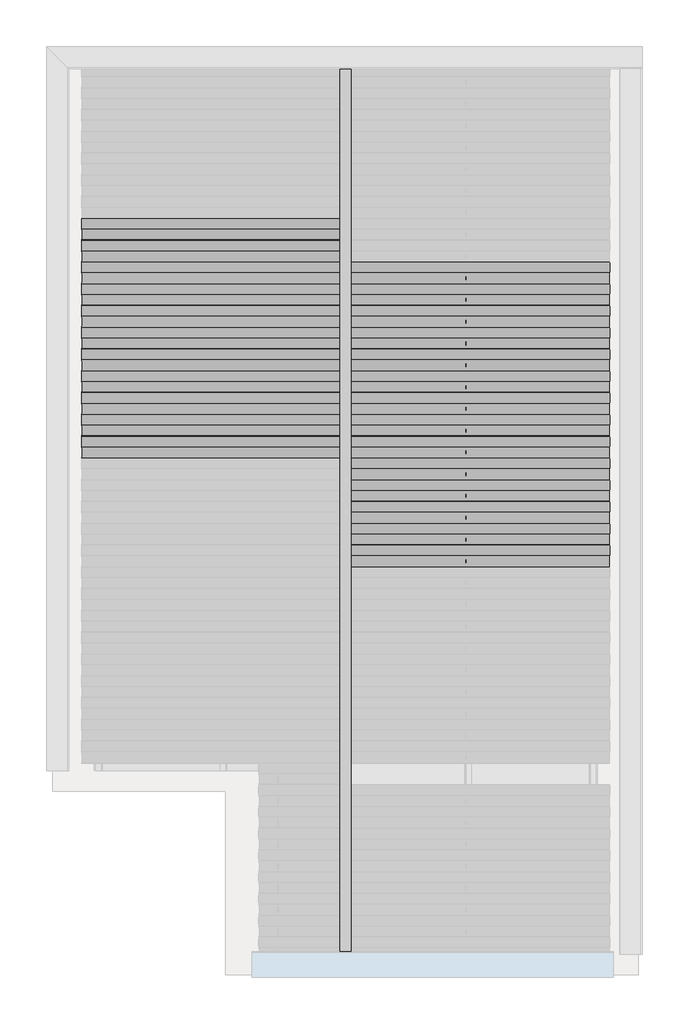
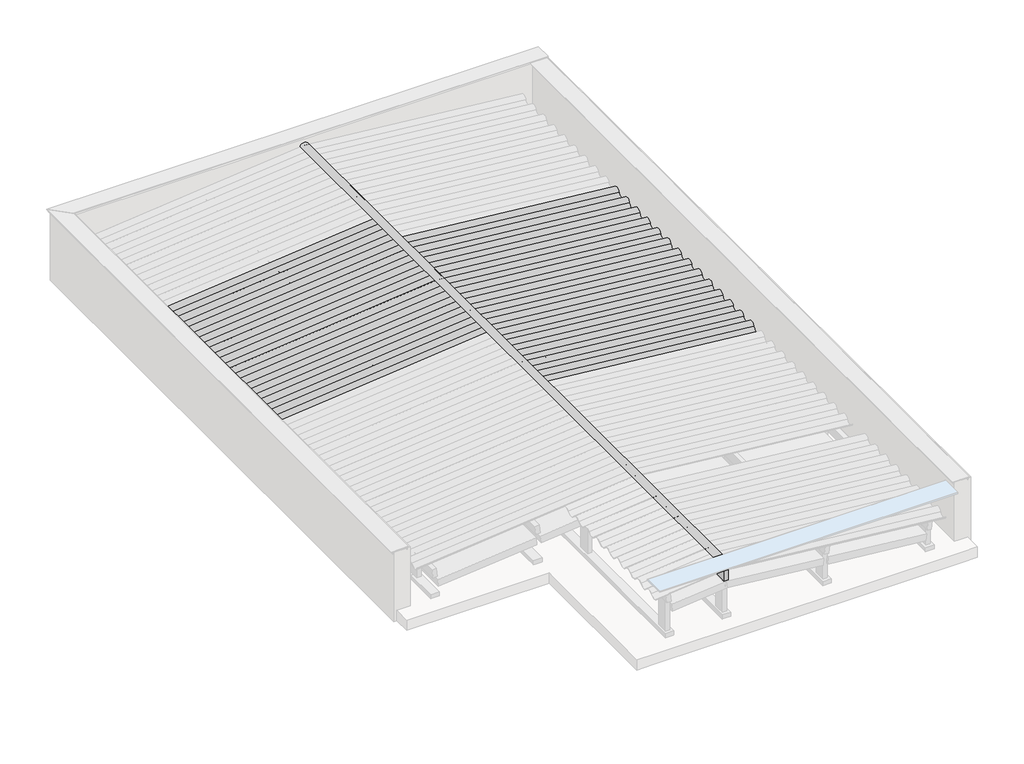
# One storey, part 3 of 4: 34 beams, 8 columns.
"""IFC4 building model written with IfcOpenShell, lengths in millimetres."""

import ifcopenshell
import ifcopenshell.guid

model = None  # the IFC model being written
_history = None  # IfcOwnerHistory: only IFC2X3 demands one
_inside = {}  # id of a spatial element -> (the spatial element, [elements in it])
_under = {}  # id of a project, library or spatial element -> (it, [spatial elements below it])
_declared = {}  # id of a project -> (the project, [libraries it declares])
_typed = {}  # id of a type object -> (the type object, [elements of that type])
_made_of = {}  # id of a material, layer set ... -> (it, [elements and type objects made of it])


def new_model(schema):
    """Start an empty IFC model of exactly this schema.

    Asked for "IFC4X3", IfcOpenShell would pick the latest addendum, in which some entities
    have other attributes; the version numbers below select the first issue.
    IFC2X3 requires an IfcOwnerHistory on every rooted entity: one is made here for all.
    """
    global model, _history
    if schema == "IFC4X3":
        model = ifcopenshell.file(schema_version=(4, 3, 0, 0))
    else:
        model = ifcopenshell.file(schema=schema)
    _inside.clear()
    _under.clear()
    _declared.clear()
    _typed.clear()
    _made_of.clear()
    _history = None
    if model.schema == "IFC2X3":
        org = make("IfcOrganization", Name="unknown")
        user = make(
            "IfcPersonAndOrganization",
            ThePerson=make("IfcPerson", FamilyName="unknown"),
            TheOrganization=org,
        )
        app = make(
            "IfcApplication",
            ApplicationDeveloper=org,
            Version="unknown",
            ApplicationFullName="unknown",
            ApplicationIdentifier="unknown",
        )
        _history = make(
            "IfcOwnerHistory",
            OwningUser=user,
            OwningApplication=app,
            ChangeAction="ADDED",
            CreationDate=0,
        )
    return model


def make(cls, **values):
    """One entity of the class cls with the attributes given. An attribute that is None is left unset."""
    return model.create_entity(
        cls, **{name: value for name, value in values.items() if value is not None}
    )


def rooted(cls, **values):
    """An entity with a GlobalId (a new one), such as an element, a storey or a relation."""
    return make(cls, GlobalId=ifcopenshell.guid.new(), OwnerHistory=_history, **values)


def si_unit(unit_type, name, prefix=None):
    """IfcSIUnit, for example si_unit("LENGTHUNIT", "METRE", prefix="MILLI")."""
    return make("IfcSIUnit", UnitType=unit_type, Prefix=prefix, Name=name)


def assignment(units):
    """IfcUnitAssignment: the units of a project."""
    return None if units is None else make("IfcUnitAssignment", Units=units)


def point(xyz):
    """IfcCartesianPoint."""
    return None if xyz is None else make("IfcCartesianPoint", Coordinates=xyz)


def direction(xyz):
    """IfcDirection."""
    return None if xyz is None else make("IfcDirection", DirectionRatios=xyz)


def frame(location, z_axis=None, x_axis=None):
    """IfcAxis2Placement3D, a coordinate frame: its origin and axes. An axis left out is left unset."""
    return make(
        "IfcAxis2Placement3D",
        Location=point(location),
        Axis=direction(z_axis),
        RefDirection=direction(x_axis),
    )


def frame_2d(location, x_axis=None):
    """IfcAxis2Placement2D, a coordinate frame in the plane: its origin and x axis."""
    return make(
        "IfcAxis2Placement2D", Location=point(location), RefDirection=direction(x_axis)
    )


def origin():
    """The frame at (0, 0, 0) with its axes left unset."""
    return frame((0.0, 0.0, 0.0))


def place(relative_to, where):
    """IfcLocalPlacement: puts the frame where relative to a parent placement (None: the world)."""
    return make(
        "IfcLocalPlacement", PlacementRelTo=relative_to, RelativePlacement=where
    )


def context(
    kind, dimensions, precision=None, world=None, true_north=None, identifier=None
):
    """IfcGeometricRepresentationContext, for example the 3D "Model" context."""
    return make(
        "IfcGeometricRepresentationContext",
        ContextIdentifier=identifier,
        ContextType=kind,
        CoordinateSpaceDimension=dimensions,
        Precision=precision,
        WorldCoordinateSystem=world,
        TrueNorth=true_north,
    )


def project(units=None, contexts=None):
    """IfcProject with its units and contexts."""
    return rooted(
        "IfcProject",
        Name="project",
        RepresentationContexts=contexts,
        UnitsInContext=assignment(units),
    )


def spatial(cls, under=None, at=None, **own):
    """A site, building, storey or space (cls), placed at a placement, below another one or the project."""
    s = rooted(cls, ObjectPlacement=at, **own)
    if under is not None:
        _under.setdefault(under.id(), (under, []))[1].append(s)
    return s


def polyline(points):
    """IfcPolyline through the points."""
    return make("IfcPolyline", Points=[point(p) for p in points])


def circle_curve(where, radius):
    """IfcCircle in the frame where."""
    return make("IfcCircle", Position=where, Radius=radius)


def trimmed(basis, trim1, trim2, sense, master):
    """IfcTrimmedCurve: the piece of a basis curve between two trims."""
    return make(
        "IfcTrimmedCurve",
        BasisCurve=basis,
        Trim1=trim1,
        Trim2=trim2,
        SenseAgreement=sense,
        MasterRepresentation=master,
    )


def segment(curve, same_sense, transition):
    """IfcCompositeCurveSegment."""
    return make(
        "IfcCompositeCurveSegment",
        Transition=transition,
        SameSense=same_sense,
        ParentCurve=curve,
    )


def composite_curve(segments, self_intersect=None):
    """IfcCompositeCurve: segments joined end to end."""
    return make("IfcCompositeCurve", Segments=segments, SelfIntersect=self_intersect)


def outline(outer, holes=None, kind="AREA"):
    """IfcArbitraryClosedProfileDef: a profile drawn as a closed curve; with holes, ...WithVoids."""
    if holes is None:
        return make("IfcArbitraryClosedProfileDef", ProfileType=kind, OuterCurve=outer)
    return make(
        "IfcArbitraryProfileDefWithVoids",
        ProfileType=kind,
        OuterCurve=outer,
        InnerCurves=holes,
    )


def extrude(swept, where, along, depth):
    """IfcExtrudedAreaSolid: the profile swept, set in the frame where, extruded along a direction by depth."""
    return make(
        "IfcExtrudedAreaSolid",
        SweptArea=swept,
        Position=where,
        ExtrudedDirection=direction(along),
        Depth=depth,
    )


def shape(context_of_items, identifier, shape_type, items):
    """IfcShapeRepresentation: the items that make up one representation, for example the "Body"."""
    return make(
        "IfcShapeRepresentation",
        ContextOfItems=context_of_items,
        RepresentationIdentifier=identifier,
        RepresentationType=shape_type,
        Items=items,
    )


def source(mapping_origin, context_of_items, identifier, shape_type, items):
    """IfcRepresentationMap: a shape defined once, which mapped items show again and again."""
    return make(
        "IfcRepresentationMap",
        MappingOrigin=mapping_origin,
        MappedRepresentation=shape(context_of_items, identifier, shape_type, items),
    )


def transform(
    local_origin,
    x_axis=None,
    y_axis=None,
    z_axis=None,
    scale=None,
    scale2=None,
    scale3=None,
    uniform=True,
):
    """IfcCartesianTransformationOperator3D, or its non-uniform kind. x_axis, y_axis, z_axis: its Axis1, 2, 3."""
    if uniform:
        return make(
            "IfcCartesianTransformationOperator3D",
            Axis1=direction(x_axis),
            Axis2=direction(y_axis),
            LocalOrigin=point(local_origin),
            Scale=scale,
            Axis3=direction(z_axis),
        )
    return make(
        "IfcCartesianTransformationOperator3DnonUniform",
        Axis1=direction(x_axis),
        Axis2=direction(y_axis),
        LocalOrigin=point(local_origin),
        Scale=scale,
        Axis3=direction(z_axis),
        Scale2=scale2,
        Scale3=scale3,
    )


def mapped(mapping_source, mapping_target):
    """IfcMappedItem: shows the shape of a source again, moved by a transform."""
    return make(
        "IfcMappedItem", MappingSource=mapping_source, MappingTarget=mapping_target
    )


def made_of(thing, what):
    """Note that an element or type object is made of a material, layer set ...; save() writes the relation."""
    if what is not None:
        _made_of.setdefault(what.id(), (what, []))[1].append(thing)
    return thing


def element(
    cls,
    number,
    at=None,
    inside=None,
    cuts=None,
    type_object=None,
    material=None,
    context=None,
    identifier="Body",
    shape_type=None,
    held_by="IfcProductDefinitionShape",
    body=None,
    shapes=None,
    **own,
):
    """One element of the class cls, such as IfcWall. Its Tag is "e" and its number.

    at: its placement. inside: the storey or other place that contains it. cuts: it is an
    opening in that element (IfcRelVoidsElement). A single representation is given by context,
    identifier, shape_type and body (its items); several are given by shapes. held_by: the class
    of the entity that holds the representations. save() writes the other relations.
    """
    e = rooted(cls, Tag="e%d" % number, ObjectPlacement=at, **own)
    if body is not None:
        shapes = [shape(context, identifier, shape_type, body)]
    if shapes is not None:
        e.Representation = make(held_by, Representations=shapes)
    if inside is not None:
        _inside.setdefault(inside.id(), (inside, []))[1].append(e)
    if cuts is not None:
        rooted(
            "IfcRelVoidsElement", RelatingBuildingElement=cuts, RelatedOpeningElement=e
        )
    if type_object is not None:
        _typed.setdefault(type_object.id(), (type_object, []))[1].append(e)
    return made_of(e, material)


def aggregate(whole, parts):
    """IfcRelAggregates: a whole, such as a stair, and the parts it consists of."""
    return rooted("IfcRelAggregates", RelatingObject=whole, RelatedObjects=parts)


def save(model, path):
    """Write the relations noted so far, then the file.

    IfcRelAggregates (storeys below a building ...), IfcRelContainedInSpatialStructure (elements
    in a storey), IfcRelDefinesByType, IfcRelAssociatesMaterial and IfcRelDeclares: one each for
    every whole, place, type object, material and project.
    """
    for whole, parts in _under.values():
        aggregate(whole, parts)
    for where, things in _inside.values():
        rooted(
            "IfcRelContainedInSpatialStructure",
            RelatedElements=things,
            RelatingStructure=where,
        )
    for kind, things in _typed.values():
        rooted("IfcRelDefinesByType", RelatedObjects=things, RelatingType=kind)
    for what, things in _made_of.values():
        rooted("IfcRelAssociatesMaterial", RelatedObjects=things, RelatingMaterial=what)
    for by, libraries in _declared.values():
        rooted("IfcRelDeclares", RelatingContext=by, RelatedDefinitions=libraries)
    model.write(path)


def cumeeira_telha_ondulada_fibrocimento_c9eafb3e(model_context):
    return source(origin(), model_context, "Body", "SweptSolid", [
        extrude(outline(composite_curve([segment(polyline([(58.3970135, 42.4437972), (53.9055884, 40.2467307)]), True, "CONTINUOUS"), segment(trimmed(circle_curve(frame_2d((-1.6029865, 13.0936483)), 61.7939461), [point((53.9055884, 40.2467307))], [point((-57.1115615, 40.2467307))], True, "CARTESIAN"), True, "CONTINUOUS"), segment(polyline([(-57.1115615, 40.2467307), (-61.6029865, 42.4437972)]), True, "CONTINUOUS"), segment(trimmed(circle_curve(frame_2d((-1.6029865, 13.0936483)), 66.7939461), [point((-61.6029865, 42.4437972))], [point((58.3970135, 42.4437972))], False, "CARTESIAN"), True, "CONTINUOUS")], self_intersect=False)), frame((-4969.5, 0.0, 0.0), z_axis=(1.0, 0.0, 0.0), x_axis=(0.0, 1.0, 0.0)), (0.0, 0.0, 1.0), 9939.0),
    ])


def viga_cumeeira_6x16cm_10b61863(model_context):
    return source(origin(), model_context, "Body", "SweptSolid", [
        extrude(outline(polyline([(4969.4999994, 30.0), (4969.4999994, -30.0), (-4969.4999994, -30.0), (-4969.4999994, 30.0), (4969.4999994, 30.0)])), frame((0.0, 0.0, -80.0), z_axis=(0.0, 0.0, 1.0), x_axis=(1.0, 0.0, 0.0)), (0.0, 0.0, 1.0), 160.0),
    ])


def column_7d6827b5(model_context):
    return source(origin(), model_context, "Body", "SweptSolid", [
        extrude(outline(polyline([(30.0, 80.0), (30.0, -80.0), (-30.0, -80.0), (-30.0, 80.0), (30.0, 80.0)])), frame((0.0, 0.0, 4460.0), z_axis=(0.0, 0.0, 1.0), x_axis=(1.0, 0.0, 0.0)), (0.0, 0.0, 1.0), 466.0),
    ])


def column_c7348c99(model_context):
    return source(origin(), model_context, "Body", "SweptSolid", [
        extrude(outline(polyline([(30.0, 80.0), (30.0, -80.0), (-30.0, -80.0), (-30.0, 80.0), (30.0, 80.0)])), frame((0.0, 0.0, 4460.0), z_axis=(0.0, 0.0, 1.0), x_axis=(1.0, 0.0, 0.0)), (0.0, 0.0, 1.0), 372.8),
    ])


def column_6cc9e01b(model_context):
    return source(origin(), model_context, "Body", "SweptSolid", [
        extrude(outline(polyline([(30.0, 80.0), (30.0, -80.0), (-30.0, -80.0), (-30.0, 80.0), (30.0, 80.0)])), frame((0.0, 0.0, 4460.0), z_axis=(0.0, 0.0, 1.0), x_axis=(1.0, 0.0, 0.0)), (0.0, 0.0, 1.0), 233.0),
    ])


model = new_model("IFC4")

# Units and contexts
model_context = context("Model", 3, world=origin())
ifc_project = project(units=[si_unit("LENGTHUNIT", "METRE", prefix="MILLI")], contexts=[model_context])

# Site, building, storey
site = spatial("IfcSite", under=ifc_project)
building = spatial("IfcBuilding", under=site)
storey = spatial("IfcBuildingStorey", under=building, Name="COB. SALA ESTAR", Elevation=4400.0)

# Beams
placement = place(None, origin())
element("IfcBeam", 1, ObjectType="Madeira de lei : Berço 6x12cm", at=placement, inside=storey, context=model_context, shape_type="SweptSolid", body=[
    extrude(outline(polyline([(-3400.8557491, 2180.4300147), (-3280.8557491, 2180.4300147), (-3280.8557491, 180.4300153), (-3400.8557491, 180.4300153), (-3400.8557491, 2180.4300147)])), frame((0.0, 0.0, 4400.0), z_axis=(0.0, 0.0, 1.0), x_axis=(1.0, 0.0, 0.0)), (0.0, 0.0, 1.0), 60.0),
])
element("IfcBeam", 2, ObjectType="Madeira de lei : Berço 6x12cm", at=placement, inside=storey, context=model_context, shape_type="SweptSolid", body=[
    extrude(outline(polyline([(-3400.8557491, 4180.4300153), (-3280.8557491, 4180.4300153), (-3280.8557491, 2180.4300159), (-3400.8557491, 2180.4300159), (-3400.8557491, 4180.4300153)])), frame((0.0, 0.0, 4400.0), z_axis=(0.0, 0.0, 1.0), x_axis=(1.0, 0.0, 0.0)), (0.0, 0.0, 1.0), 60.0),
])
element("IfcBeam", 3, ObjectType="Madeira de lei : Berço 6x12cm", at=placement, inside=storey, context=model_context, shape_type="SweptSolid", body=[
    extrude(outline(polyline([(-2032.3324227, 2180.4300147), (-1912.3324227, 2180.4300147), (-1912.3324227, 180.4300153), (-2032.3324227, 180.4300153), (-2032.3324227, 2180.4300147)])), frame((0.0, 0.0, 4400.0), z_axis=(0.0, 0.0, 1.0), x_axis=(1.0, 0.0, 0.0)), (0.0, 0.0, 1.0), 60.0),
])
element("IfcBeam", 4, ObjectType="Madeira de lei : Berço 6x12cm", at=placement, inside=storey, context=model_context, shape_type="SweptSolid", body=[
    extrude(outline(polyline([(-634.0324227, 2180.4300147), (-514.0324227, 2180.4300147), (-514.0324227, 180.4300153), (-634.0324227, 180.4300153), (-634.0324227, 2180.4300147)])), frame((0.0, 0.0, 4400.0), z_axis=(0.0, 0.0, 1.0), x_axis=(1.0, 0.0, 0.0)), (0.0, 0.0, 1.0), 60.0),
])
element("IfcBeam", 5, ObjectType="Madeira de lei : Berço 6x12cm", at=placement, inside=storey, context=model_context, shape_type="SweptSolid", body=[
    extrude(outline(polyline([(-6167.5301913, 4180.4300153), (-6047.5301913, 4180.4300153), (-6047.5301913, 2180.4300159), (-6167.5301913, 2180.4300159), (-6167.5301913, 4180.4300153)])), frame((0.0, 0.0, 4400.0), z_axis=(0.0, 0.0, 1.0), x_axis=(1.0, 0.0, 0.0)), (0.0, 0.0, 1.0), 60.0),
])
element("IfcBeam", 6, ObjectType="Madeira de lei : Berço 6x12cm", at=placement, inside=storey, context=model_context, shape_type="SweptSolid", body=[
    extrude(outline(polyline([(-4769.2301913, 2180.4300147), (-4649.2301913, 2180.4300147), (-4649.2301913, 180.4300153), (-4769.2301913, 180.4300153), (-4769.2301913, 2180.4300147)])), frame((0.0, 0.0, 4400.0), z_axis=(0.0, 0.0, 1.0), x_axis=(1.0, 0.0, 0.0)), (0.0, 0.0, 1.0), 60.0),
])
element("IfcBeam", 7, ObjectType="Madeira de lei : Berço 6x12cm", at=placement, inside=storey, context=model_context, shape_type="SweptSolid", body=[
    extrude(outline(polyline([(-4769.2301913, 4180.4300153), (-4649.2301913, 4180.4300153), (-4649.2301913, 2180.4300159), (-4769.2301913, 2180.4300159), (-4769.2301913, 4180.4300153)])), frame((0.0, 0.0, 4400.0), z_axis=(0.0, 0.0, 1.0), x_axis=(1.0, 0.0, 0.0)), (0.0, 0.0, 1.0), 60.0),
])
cumeeira_telha_ondulada_fibrocimento_shape = cumeeira_telha_ondulada_fibrocimento_c9eafb3e(model_context)
element("IfcBeam", 8, ObjectType="Cumeeira Telha Ondulada : Fibrocimento", at=placement, inside=storey, context=model_context, shape_type="MappedRepresentation", body=[
    mapped(cumeeira_telha_ondulada_fibrocimento_shape, transform((-3340.8557491, 623.9300153, 5123.1251229), x_axis=(0.0, -1.0, 0.0), y_axis=(1.0, 0.0, 0.0), z_axis=(0.0, 0.0, 1.0))),
])
element("IfcBeam", 9, ObjectType="Telha Ondulada : Fibrocimento", at=placement, inside=storey, context=model_context, shape_type="SweptSolid", body=[
    extrude(outline(composite_curve([segment(trimmed(circle_curve(frame_2d((-58.7002978, -53.2060538)), 66.7939461), [point((-29.3501489, 6.7939462))], [point((-29.3501489, -113.2060538))], False, "CARTESIAN"), True, "CONTINUOUS"), segment(polyline([(-29.3501489, -113.2060538), (-31.5472154, -108.7146288)]), True, "CONTINUOUS"), segment(trimmed(circle_curve(frame_2d((-58.7002978, -53.2060538)), 61.7939461), [point((-31.5472154, -108.7146288))], [point((-31.5472154, 2.3025211))], True, "CARTESIAN"), True, "CONTINUOUS"), segment(trimmed(circle_curve(frame_2d((0.0, 66.7939462)), 71.7939461), [point((-31.5472154, 2.3025211))], [point((-31.5472154, 131.2853712))], False, "CARTESIAN"), True, "CONTINUOUS"), segment(polyline([(-31.5472154, 131.2853712), (-29.3501489, 126.7939462)]), True, "CONTINUOUS"), segment(trimmed(circle_curve(frame_2d((0.0, 66.7939462)), 66.7939461), [point((-29.3501489, 126.7939462))], [point((-29.3501489, 6.7939462))], True, "CARTESIAN"), True, "CONTINUOUS")], self_intersect=False)), frame((-6307.6707245, 1355.826948, 4862.7215886), z_axis=(0.9950371902099892, 0.0, 0.09950371902099969), x_axis=(-0.09950371902099969, 0.0, 0.9950371902099892)), (0.0, 0.0, 1.0), 2972.5075682),
])
element("IfcBeam", 10, ObjectType="Telha Ondulada : Fibrocimento", at=placement, inside=storey, context=model_context, shape_type="SweptSolid", body=[
    extrude(outline(composite_curve([segment(trimmed(circle_curve(frame_2d((-58.7002978, -53.2060538)), 66.7939461), [point((-29.3501489, 6.7939462))], [point((-29.3501489, -113.2060538))], False, "CARTESIAN"), True, "CONTINUOUS"), segment(polyline([(-29.3501489, -113.2060538), (-31.5472154, -108.7146288)]), True, "CONTINUOUS"), segment(trimmed(circle_curve(frame_2d((-58.7002978, -53.2060538)), 61.7939461), [point((-31.5472154, -108.7146288))], [point((-31.5472154, 2.3025211))], True, "CARTESIAN"), True, "CONTINUOUS"), segment(trimmed(circle_curve(frame_2d((0.0, 66.7939462)), 71.7939461), [point((-31.5472154, 2.3025211))], [point((-31.5472154, 131.2853712))], False, "CARTESIAN"), True, "CONTINUOUS"), segment(polyline([(-31.5472154, 131.2853712), (-29.3501489, 126.7939462)]), True, "CONTINUOUS"), segment(trimmed(circle_curve(frame_2d((0.0, 66.7939462)), 66.7939461), [point((-29.3501489, 126.7939462))], [point((-29.3501489, 6.7939462))], True, "CARTESIAN"), True, "CONTINUOUS")], self_intersect=False)), frame((-6307.6707245, 1600.326948, 4862.7215886), z_axis=(0.9950371902099892, 0.0, 0.09950371902099972), x_axis=(-0.09950371902099972, 0.0, 0.9950371902099892)), (0.0, 0.0, 1.0), 2972.5075682),
])
element("IfcBeam", 11, ObjectType="Telha Ondulada : Fibrocimento", at=placement, inside=storey, context=model_context, shape_type="SweptSolid", body=[
    extrude(outline(composite_curve([segment(trimmed(circle_curve(frame_2d((-58.7002978, -53.2060538)), 66.7939461), [point((-29.3501489, 6.7939462))], [point((-29.3501489, -113.2060538))], False, "CARTESIAN"), True, "CONTINUOUS"), segment(polyline([(-29.3501489, -113.2060538), (-31.5472154, -108.7146288)]), True, "CONTINUOUS"), segment(trimmed(circle_curve(frame_2d((-58.7002978, -53.2060538)), 61.7939461), [point((-31.5472154, -108.7146288))], [point((-31.5472154, 2.3025211))], True, "CARTESIAN"), True, "CONTINUOUS"), segment(trimmed(circle_curve(frame_2d((0.0, 66.7939462)), 71.7939461), [point((-31.5472154, 2.3025211))], [point((-31.5472154, 131.2853712))], False, "CARTESIAN"), True, "CONTINUOUS"), segment(polyline([(-31.5472154, 131.2853712), (-29.3501489, 126.7939462)]), True, "CONTINUOUS"), segment(trimmed(circle_curve(frame_2d((0.0, 66.7939462)), 66.7939461), [point((-29.3501489, 126.7939462))], [point((-29.3501489, 6.7939462))], True, "CARTESIAN"), True, "CONTINUOUS")], self_intersect=False)), frame((-6307.6707245, 1844.826948, 4862.7215886), z_axis=(0.9950371902099892, 0.0, 0.09950371902099972), x_axis=(-0.09950371902099972, 0.0, 0.9950371902099892)), (0.0, 0.0, 1.0), 2972.5075682),
])
element("IfcBeam", 12, ObjectType="Telha Ondulada : Fibrocimento", at=placement, inside=storey, context=model_context, shape_type="SweptSolid", body=[
    extrude(outline(composite_curve([segment(trimmed(circle_curve(frame_2d((-58.7002978, -53.2060538)), 66.7939461), [point((-29.3501489, 6.7939462))], [point((-29.3501489, -113.2060538))], False, "CARTESIAN"), True, "CONTINUOUS"), segment(polyline([(-29.3501489, -113.2060538), (-31.5472154, -108.7146288)]), True, "CONTINUOUS"), segment(trimmed(circle_curve(frame_2d((-58.7002978, -53.2060538)), 61.7939461), [point((-31.5472154, -108.7146288))], [point((-31.5472154, 2.3025211))], True, "CARTESIAN"), True, "CONTINUOUS"), segment(trimmed(circle_curve(frame_2d((0.0, 66.7939462)), 71.7939461), [point((-31.5472154, 2.3025211))], [point((-31.5472154, 131.2853712))], False, "CARTESIAN"), True, "CONTINUOUS"), segment(polyline([(-31.5472154, 131.2853712), (-29.3501489, 126.7939462)]), True, "CONTINUOUS"), segment(trimmed(circle_curve(frame_2d((0.0, 66.7939462)), 66.7939461), [point((-29.3501489, 126.7939462))], [point((-29.3501489, 6.7939462))], True, "CARTESIAN"), True, "CONTINUOUS")], self_intersect=False)), frame((-6307.6707245, 2089.326948, 4862.7215886), z_axis=(0.9950371902099892, 0.0, 0.09950371902099954), x_axis=(-0.09950371902099954, 0.0, 0.9950371902099892)), (0.0, 0.0, 1.0), 2972.5075682),
])
element("IfcBeam", 13, ObjectType="Telha Ondulada : Fibrocimento", at=placement, inside=storey, context=model_context, shape_type="SweptSolid", body=[
    extrude(outline(composite_curve([segment(trimmed(circle_curve(frame_2d((-58.7002978, -53.2060538)), 66.7939461), [point((-29.3501489, 6.7939462))], [point((-29.3501489, -113.2060538))], False, "CARTESIAN"), True, "CONTINUOUS"), segment(polyline([(-29.3501489, -113.2060538), (-31.5472154, -108.7146288)]), True, "CONTINUOUS"), segment(trimmed(circle_curve(frame_2d((-58.7002978, -53.2060538)), 61.7939461), [point((-31.5472154, -108.7146288))], [point((-31.5472154, 2.3025211))], True, "CARTESIAN"), True, "CONTINUOUS"), segment(trimmed(circle_curve(frame_2d((0.0, 66.7939462)), 71.7939461), [point((-31.5472154, 2.3025211))], [point((-31.5472154, 131.2853712))], False, "CARTESIAN"), True, "CONTINUOUS"), segment(polyline([(-31.5472154, 131.2853712), (-29.3501489, 126.7939462)]), True, "CONTINUOUS"), segment(trimmed(circle_curve(frame_2d((0.0, 66.7939462)), 66.7939461), [point((-29.3501489, 126.7939462))], [point((-29.3501489, 6.7939462))], True, "CARTESIAN"), True, "CONTINUOUS")], self_intersect=False)), frame((-6307.6707245, 2333.826948, 4862.7215886), z_axis=(0.9950371902099892, 0.0, 0.09950371902099972), x_axis=(-0.09950371902099972, 0.0, 0.9950371902099892)), (0.0, 0.0, 1.0), 2972.5075682),
])
element("IfcBeam", 14, ObjectType="Telha Ondulada : Fibrocimento", at=placement, inside=storey, context=model_context, shape_type="SweptSolid", body=[
    extrude(outline(composite_curve([segment(trimmed(circle_curve(frame_2d((-58.7002978, -53.2060538)), 66.7939461), [point((-29.3501489, 6.7939462))], [point((-29.3501489, -113.2060538))], False, "CARTESIAN"), True, "CONTINUOUS"), segment(polyline([(-29.3501489, -113.2060538), (-31.5472154, -108.7146288)]), True, "CONTINUOUS"), segment(trimmed(circle_curve(frame_2d((-58.7002978, -53.2060538)), 61.7939461), [point((-31.5472154, -108.7146288))], [point((-31.5472154, 2.3025211))], True, "CARTESIAN"), True, "CONTINUOUS"), segment(trimmed(circle_curve(frame_2d((0.0, 66.7939462)), 71.7939461), [point((-31.5472154, 2.3025211))], [point((-31.5472154, 131.2853712))], False, "CARTESIAN"), True, "CONTINUOUS"), segment(polyline([(-31.5472154, 131.2853712), (-29.3501489, 126.7939462)]), True, "CONTINUOUS"), segment(trimmed(circle_curve(frame_2d((0.0, 66.7939462)), 66.7939461), [point((-29.3501489, 126.7939462))], [point((-29.3501489, 6.7939462))], True, "CARTESIAN"), True, "CONTINUOUS")], self_intersect=False)), frame((-6307.6707245, 2578.326948, 4862.7215886), z_axis=(0.9950371902099892, 0.0, 0.09950371902099969), x_axis=(-0.09950371902099969, 0.0, 0.9950371902099892)), (0.0, 0.0, 1.0), 2972.5075682),
])
element("IfcBeam", 15, ObjectType="Telha Ondulada : Fibrocimento", at=placement, inside=storey, context=model_context, shape_type="SweptSolid", body=[
    extrude(outline(composite_curve([segment(trimmed(circle_curve(frame_2d((-58.7002978, -53.2060538)), 66.7939461), [point((-29.3501489, 6.7939462))], [point((-29.3501489, -113.2060538))], False, "CARTESIAN"), True, "CONTINUOUS"), segment(polyline([(-29.3501489, -113.2060538), (-31.5472154, -108.7146288)]), True, "CONTINUOUS"), segment(trimmed(circle_curve(frame_2d((-58.7002978, -53.2060538)), 61.7939461), [point((-31.5472154, -108.7146288))], [point((-31.5472154, 2.3025211))], True, "CARTESIAN"), True, "CONTINUOUS"), segment(trimmed(circle_curve(frame_2d((0.0, 66.7939462)), 71.7939461), [point((-31.5472154, 2.3025211))], [point((-31.5472154, 131.2853712))], False, "CARTESIAN"), True, "CONTINUOUS"), segment(polyline([(-31.5472154, 131.2853712), (-29.3501489, 126.7939462)]), True, "CONTINUOUS"), segment(trimmed(circle_curve(frame_2d((0.0, 66.7939462)), 66.7939461), [point((-29.3501489, 126.7939462))], [point((-29.3501489, 6.7939462))], True, "CARTESIAN"), True, "CONTINUOUS")], self_intersect=False)), frame((-6307.6707245, 2822.826948, 4862.7215886), z_axis=(0.9950371902099892, 0.0, 0.09950371902099972), x_axis=(-0.09950371902099972, 0.0, 0.9950371902099892)), (0.0, 0.0, 1.0), 2972.5075682),
])
element("IfcBeam", 16, ObjectType="Telha Ondulada : Fibrocimento", at=placement, inside=storey, context=model_context, shape_type="SweptSolid", body=[
    extrude(outline(composite_curve([segment(trimmed(circle_curve(frame_2d((-58.7002978, -53.2060538)), 66.7939461), [point((-29.3501489, 6.7939462))], [point((-29.3501489, -113.2060538))], False, "CARTESIAN"), True, "CONTINUOUS"), segment(polyline([(-29.3501489, -113.2060538), (-31.5472154, -108.7146288)]), True, "CONTINUOUS"), segment(trimmed(circle_curve(frame_2d((-58.7002978, -53.2060538)), 61.7939461), [point((-31.5472154, -108.7146288))], [point((-31.5472154, 2.3025211))], True, "CARTESIAN"), True, "CONTINUOUS"), segment(trimmed(circle_curve(frame_2d((0.0, 66.7939462)), 71.7939461), [point((-31.5472154, 2.3025211))], [point((-31.5472154, 131.2853712))], False, "CARTESIAN"), True, "CONTINUOUS"), segment(polyline([(-31.5472154, 131.2853712), (-29.3501489, 126.7939462)]), True, "CONTINUOUS"), segment(trimmed(circle_curve(frame_2d((0.0, 66.7939462)), 66.7939461), [point((-29.3501489, 126.7939462))], [point((-29.3501489, 6.7939462))], True, "CARTESIAN"), True, "CONTINUOUS")], self_intersect=False)), frame((-6307.6707245, 3067.326948, 4862.7215886), z_axis=(0.9950371902099892, 0.0, 0.09950371902099972), x_axis=(-0.09950371902099972, 0.0, 0.9950371902099892)), (0.0, 0.0, 1.0), 2972.5075682),
])
element("IfcBeam", 17, ObjectType="Telha Ondulada : Fibrocimento", at=placement, inside=storey, context=model_context, shape_type="SweptSolid", body=[
    extrude(outline(composite_curve([segment(trimmed(circle_curve(frame_2d((-58.7002978, -53.2060538)), 66.7939461), [point((-29.3501489, 6.7939462))], [point((-29.3501489, -113.2060538))], False, "CARTESIAN"), True, "CONTINUOUS"), segment(polyline([(-29.3501489, -113.2060538), (-31.5472154, -108.7146288)]), True, "CONTINUOUS"), segment(trimmed(circle_curve(frame_2d((-58.7002978, -53.2060538)), 61.7939461), [point((-31.5472154, -108.7146288))], [point((-31.5472154, 2.3025211))], True, "CARTESIAN"), True, "CONTINUOUS"), segment(trimmed(circle_curve(frame_2d((0.0, 66.7939462)), 71.7939461), [point((-31.5472154, 2.3025211))], [point((-31.5472154, 131.2853712))], False, "CARTESIAN"), True, "CONTINUOUS"), segment(polyline([(-31.5472154, 131.2853712), (-29.3501489, 126.7939462)]), True, "CONTINUOUS"), segment(trimmed(circle_curve(frame_2d((0.0, 66.7939462)), 66.7939461), [point((-29.3501489, 126.7939462))], [point((-29.3501489, 6.7939462))], True, "CARTESIAN"), True, "CONTINUOUS")], self_intersect=False)), frame((-6307.6707245, 3311.826948, 4862.7215886), z_axis=(0.9950371902099892, 0.0, 0.09950371902099954), x_axis=(-0.09950371902099954, 0.0, 0.9950371902099892)), (0.0, 0.0, 1.0), 2972.5075682),
])
element("IfcBeam", 18, ObjectType="Telha Ondulada : Fibrocimento", at=placement, inside=storey, context=model_context, shape_type="SweptSolid", body=[
    extrude(outline(composite_curve([segment(trimmed(circle_curve(frame_2d((-58.7002978, -53.2060538)), 66.7939461), [point((-29.3501489, 6.7939462))], [point((-29.3501489, -113.2060538))], False, "CARTESIAN"), True, "CONTINUOUS"), segment(polyline([(-29.3501489, -113.2060538), (-31.5472154, -108.7146288)]), True, "CONTINUOUS"), segment(trimmed(circle_curve(frame_2d((-58.7002978, -53.2060538)), 61.7939461), [point((-31.5472154, -108.7146288))], [point((-31.5472154, 2.3025211))], True, "CARTESIAN"), True, "CONTINUOUS"), segment(trimmed(circle_curve(frame_2d((0.0, 66.7939462)), 71.7939461), [point((-31.5472154, 2.3025211))], [point((-31.5472154, 131.2853712))], False, "CARTESIAN"), True, "CONTINUOUS"), segment(polyline([(-31.5472154, 131.2853712), (-29.3501489, 126.7939462)]), True, "CONTINUOUS"), segment(trimmed(circle_curve(frame_2d((0.0, 66.7939462)), 66.7939461), [point((-29.3501489, 126.7939462))], [point((-29.3501489, 6.7939462))], True, "CARTESIAN"), True, "CONTINUOUS")], self_intersect=False)), frame((-6307.6707245, 3556.326948, 4862.7215886), z_axis=(0.9950371902099892, 0.0, 0.09950371902099954), x_axis=(-0.09950371902099954, 0.0, 0.9950371902099892)), (0.0, 0.0, 1.0), 2972.5075682),
])
element("IfcBeam", 19, ObjectType="Telha Ondulada : Fibrocimento", at=placement, inside=storey, context=model_context, shape_type="SweptSolid", body=[
    extrude(outline(composite_curve([segment(trimmed(circle_curve(frame_2d((-58.7002978, -53.2060538)), 66.7939461), [point((-29.3501489, 6.7939462))], [point((-29.3501489, -113.2060538))], False, "CARTESIAN"), True, "CONTINUOUS"), segment(polyline([(-29.3501489, -113.2060538), (-31.5472154, -108.7146288)]), True, "CONTINUOUS"), segment(trimmed(circle_curve(frame_2d((-58.7002978, -53.2060538)), 61.7939461), [point((-31.5472154, -108.7146288))], [point((-31.5472154, 2.3025211))], True, "CARTESIAN"), True, "CONTINUOUS"), segment(trimmed(circle_curve(frame_2d((0.0, 66.7939462)), 71.7939461), [point((-31.5472154, 2.3025211))], [point((-31.5472154, 131.2853712))], False, "CARTESIAN"), True, "CONTINUOUS"), segment(polyline([(-31.5472154, 131.2853712), (-29.3501489, 126.7939462)]), True, "CONTINUOUS"), segment(trimmed(circle_curve(frame_2d((0.0, 66.7939462)), 66.7939461), [point((-29.3501489, 126.7939462))], [point((-29.3501489, 6.7939462))], True, "CARTESIAN"), True, "CONTINUOUS")], self_intersect=False)), frame((-6307.6707245, 3800.826948, 4862.7215886), z_axis=(0.9950371902099892, 0.0, 0.09950371902099968), x_axis=(-0.09950371902099968, 0.0, 0.9950371902099892)), (0.0, 0.0, 1.0), 2972.5075682),
])
element("IfcBeam", 20, ObjectType="Telha Ondulada : Fibrocimento", at=placement, inside=storey, context=model_context, shape_type="SweptSolid", body=[
    extrude(outline(composite_curve([segment(trimmed(circle_curve(frame_2d((0.0, 66.7939462)), 66.7939461), [point((29.3501489, 6.7939462))], [point((29.3501489, 126.7939462))], True, "CARTESIAN"), True, "CONTINUOUS"), segment(polyline([(29.3501489, 126.7939462), (31.5472154, 131.2853712)]), True, "CONTINUOUS"), segment(trimmed(circle_curve(frame_2d((0.0, 66.7939462)), 71.7939461), [point((31.5472154, 131.2853712))], [point((31.5472154, 2.3025211))], False, "CARTESIAN"), True, "CONTINUOUS"), segment(trimmed(circle_curve(frame_2d((58.7002978, -53.2060538)), 61.7939461), [point((31.5472154, 2.3025211))], [point((31.5472154, -108.7146288))], True, "CARTESIAN"), True, "CONTINUOUS"), segment(polyline([(31.5472154, -108.7146288), (29.3501489, -113.2060538)]), True, "CONTINUOUS"), segment(trimmed(circle_curve(frame_2d((58.7002978, -53.2060538)), 66.7939461), [point((29.3501489, -113.2060538))], [point((29.3501489, 6.7939462))], False, "CARTESIAN"), True, "CONTINUOUS")], self_intersect=False)), frame((-373.8918894, 133.326948, 4862.7215886), z_axis=(-0.9950371902099892, 0.0, 0.09950371902099946), x_axis=(-0.09950371902099946, 0.0, -0.9950371902099892)), (0.0, 0.0, 1.0), 2972.5075682),
])
element("IfcBeam", 21, ObjectType="Telha Ondulada : Fibrocimento", at=placement, inside=storey, context=model_context, shape_type="SweptSolid", body=[
    extrude(outline(composite_curve([segment(trimmed(circle_curve(frame_2d((0.0, 66.7939462)), 66.7939461), [point((29.3501489, 6.7939462))], [point((29.3501489, 126.7939462))], True, "CARTESIAN"), True, "CONTINUOUS"), segment(polyline([(29.3501489, 126.7939462), (31.5472154, 131.2853712)]), True, "CONTINUOUS"), segment(trimmed(circle_curve(frame_2d((0.0, 66.7939462)), 71.7939461), [point((31.5472154, 131.2853712))], [point((31.5472154, 2.3025211))], False, "CARTESIAN"), True, "CONTINUOUS"), segment(trimmed(circle_curve(frame_2d((58.7002978, -53.2060538)), 61.7939461), [point((31.5472154, 2.3025211))], [point((31.5472154, -108.7146288))], True, "CARTESIAN"), True, "CONTINUOUS"), segment(polyline([(31.5472154, -108.7146288), (29.3501489, -113.2060538)]), True, "CONTINUOUS"), segment(trimmed(circle_curve(frame_2d((58.7002978, -53.2060538)), 66.7939461), [point((29.3501489, -113.2060538))], [point((29.3501489, 6.7939462))], False, "CARTESIAN"), True, "CONTINUOUS")], self_intersect=False)), frame((-373.8918894, 377.826948, 4862.7215886), z_axis=(-0.9950371902099892, 0.0, 0.09950371902099946), x_axis=(-0.09950371902099946, 0.0, -0.9950371902099892)), (0.0, 0.0, 1.0), 2972.5075682),
])
element("IfcBeam", 22, ObjectType="Telha Ondulada : Fibrocimento", at=placement, inside=storey, context=model_context, shape_type="SweptSolid", body=[
    extrude(outline(composite_curve([segment(trimmed(circle_curve(frame_2d((0.0, 66.7939462)), 66.7939461), [point((29.3501489, 6.7939462))], [point((29.3501489, 126.7939462))], True, "CARTESIAN"), True, "CONTINUOUS"), segment(polyline([(29.3501489, 126.7939462), (31.5472154, 131.2853712)]), True, "CONTINUOUS"), segment(trimmed(circle_curve(frame_2d((0.0, 66.7939462)), 71.7939461), [point((31.5472154, 131.2853712))], [point((31.5472154, 2.3025211))], False, "CARTESIAN"), True, "CONTINUOUS"), segment(trimmed(circle_curve(frame_2d((58.7002978, -53.2060538)), 61.7939461), [point((31.5472154, 2.3025211))], [point((31.5472154, -108.7146288))], True, "CARTESIAN"), True, "CONTINUOUS"), segment(polyline([(31.5472154, -108.7146288), (29.3501489, -113.2060538)]), True, "CONTINUOUS"), segment(trimmed(circle_curve(frame_2d((58.7002978, -53.2060538)), 66.7939461), [point((29.3501489, -113.2060538))], [point((29.3501489, 6.7939462))], False, "CARTESIAN"), True, "CONTINUOUS")], self_intersect=False)), frame((-373.8918894, 622.326948, 4862.7215886), z_axis=(-0.9950371902099892, 0.0, 0.09950371902099946), x_axis=(-0.09950371902099946, 0.0, -0.9950371902099892)), (0.0, 0.0, 1.0), 2972.5075682),
])
element("IfcBeam", 23, ObjectType="Telha Ondulada : Fibrocimento", at=placement, inside=storey, context=model_context, shape_type="SweptSolid", body=[
    extrude(outline(composite_curve([segment(trimmed(circle_curve(frame_2d((0.0, 66.7939462)), 66.7939461), [point((29.3501489, 6.7939462))], [point((29.3501489, 126.7939462))], True, "CARTESIAN"), True, "CONTINUOUS"), segment(polyline([(29.3501489, 126.7939462), (31.5472154, 131.2853712)]), True, "CONTINUOUS"), segment(trimmed(circle_curve(frame_2d((0.0, 66.7939462)), 71.7939461), [point((31.5472154, 131.2853712))], [point((31.5472154, 2.3025211))], False, "CARTESIAN"), True, "CONTINUOUS"), segment(trimmed(circle_curve(frame_2d((58.7002978, -53.2060538)), 61.7939461), [point((31.5472154, 2.3025211))], [point((31.5472154, -108.7146288))], True, "CARTESIAN"), True, "CONTINUOUS"), segment(polyline([(31.5472154, -108.7146288), (29.3501489, -113.2060538)]), True, "CONTINUOUS"), segment(trimmed(circle_curve(frame_2d((58.7002978, -53.2060538)), 66.7939461), [point((29.3501489, -113.2060538))], [point((29.3501489, 6.7939462))], False, "CARTESIAN"), True, "CONTINUOUS")], self_intersect=False)), frame((-373.8918894, 866.826948, 4862.7215886), z_axis=(-0.9950371902099892, 0.0, 0.09950371902099946), x_axis=(-0.09950371902099946, 0.0, -0.9950371902099892)), (0.0, 0.0, 1.0), 2972.5075682),
])
element("IfcBeam", 24, ObjectType="Telha Ondulada : Fibrocimento", at=placement, inside=storey, context=model_context, shape_type="SweptSolid", body=[
    extrude(outline(composite_curve([segment(trimmed(circle_curve(frame_2d((0.0, 66.7939462)), 66.7939461), [point((29.3501489, 6.7939462))], [point((29.3501489, 126.7939462))], True, "CARTESIAN"), True, "CONTINUOUS"), segment(polyline([(29.3501489, 126.7939462), (31.5472154, 131.2853712)]), True, "CONTINUOUS"), segment(trimmed(circle_curve(frame_2d((0.0, 66.7939462)), 71.7939461), [point((31.5472154, 131.2853712))], [point((31.5472154, 2.3025211))], False, "CARTESIAN"), True, "CONTINUOUS"), segment(trimmed(circle_curve(frame_2d((58.7002978, -53.2060538)), 61.7939461), [point((31.5472154, 2.3025211))], [point((31.5472154, -108.7146288))], True, "CARTESIAN"), True, "CONTINUOUS"), segment(polyline([(31.5472154, -108.7146288), (29.3501489, -113.2060538)]), True, "CONTINUOUS"), segment(trimmed(circle_curve(frame_2d((58.7002978, -53.2060538)), 66.7939461), [point((29.3501489, -113.2060538))], [point((29.3501489, 6.7939462))], False, "CARTESIAN"), True, "CONTINUOUS")], self_intersect=False)), frame((-373.8918894, 1111.326948, 4862.7215886), z_axis=(-0.9950371902099892, 0.0, 0.09950371902099946), x_axis=(-0.09950371902099946, 0.0, -0.9950371902099892)), (0.0, 0.0, 1.0), 2972.5075682),
])
element("IfcBeam", 25, ObjectType="Telha Ondulada : Fibrocimento", at=placement, inside=storey, context=model_context, shape_type="SweptSolid", body=[
    extrude(outline(composite_curve([segment(trimmed(circle_curve(frame_2d((0.0, 66.7939462)), 66.7939461), [point((29.3501489, 6.7939462))], [point((29.3501489, 126.7939462))], True, "CARTESIAN"), True, "CONTINUOUS"), segment(polyline([(29.3501489, 126.7939462), (31.5472154, 131.2853712)]), True, "CONTINUOUS"), segment(trimmed(circle_curve(frame_2d((0.0, 66.7939462)), 71.7939461), [point((31.5472154, 131.2853712))], [point((31.5472154, 2.3025211))], False, "CARTESIAN"), True, "CONTINUOUS"), segment(trimmed(circle_curve(frame_2d((58.7002978, -53.2060538)), 61.7939461), [point((31.5472154, 2.3025211))], [point((31.5472154, -108.7146288))], True, "CARTESIAN"), True, "CONTINUOUS"), segment(polyline([(31.5472154, -108.7146288), (29.3501489, -113.2060538)]), True, "CONTINUOUS"), segment(trimmed(circle_curve(frame_2d((58.7002978, -53.2060538)), 66.7939461), [point((29.3501489, -113.2060538))], [point((29.3501489, 6.7939462))], False, "CARTESIAN"), True, "CONTINUOUS")], self_intersect=False)), frame((-373.8918894, 1355.826948, 4862.7215886), z_axis=(-0.9950371902099892, 0.0, 0.09950371902099946), x_axis=(-0.09950371902099946, 0.0, -0.9950371902099892)), (0.0, 0.0, 1.0), 2972.5075682),
])
element("IfcBeam", 26, ObjectType="Telha Ondulada : Fibrocimento", at=placement, inside=storey, context=model_context, shape_type="SweptSolid", body=[
    extrude(outline(composite_curve([segment(trimmed(circle_curve(frame_2d((0.0, 66.7939462)), 66.7939461), [point((29.3501489, 6.7939462))], [point((29.3501489, 126.7939462))], True, "CARTESIAN"), True, "CONTINUOUS"), segment(polyline([(29.3501489, 126.7939462), (31.5472154, 131.2853712)]), True, "CONTINUOUS"), segment(trimmed(circle_curve(frame_2d((0.0, 66.7939462)), 71.7939461), [point((31.5472154, 131.2853712))], [point((31.5472154, 2.3025211))], False, "CARTESIAN"), True, "CONTINUOUS"), segment(trimmed(circle_curve(frame_2d((58.7002978, -53.2060538)), 61.7939461), [point((31.5472154, 2.3025211))], [point((31.5472154, -108.7146288))], True, "CARTESIAN"), True, "CONTINUOUS"), segment(polyline([(31.5472154, -108.7146288), (29.3501489, -113.2060538)]), True, "CONTINUOUS"), segment(trimmed(circle_curve(frame_2d((58.7002978, -53.2060538)), 66.7939461), [point((29.3501489, -113.2060538))], [point((29.3501489, 6.7939462))], False, "CARTESIAN"), True, "CONTINUOUS")], self_intersect=False)), frame((-373.8918894, 1600.326948, 4862.7215886), z_axis=(-0.9950371902099892, 0.0, 0.09950371902099946), x_axis=(-0.09950371902099946, 0.0, -0.9950371902099892)), (0.0, 0.0, 1.0), 2972.5075682),
])
element("IfcBeam", 27, ObjectType="Telha Ondulada : Fibrocimento", at=placement, inside=storey, context=model_context, shape_type="SweptSolid", body=[
    extrude(outline(composite_curve([segment(trimmed(circle_curve(frame_2d((0.0, 66.7939462)), 66.7939461), [point((29.3501489, 6.7939462))], [point((29.3501489, 126.7939462))], True, "CARTESIAN"), True, "CONTINUOUS"), segment(polyline([(29.3501489, 126.7939462), (31.5472154, 131.2853712)]), True, "CONTINUOUS"), segment(trimmed(circle_curve(frame_2d((0.0, 66.7939462)), 71.7939461), [point((31.5472154, 131.2853712))], [point((31.5472154, 2.3025211))], False, "CARTESIAN"), True, "CONTINUOUS"), segment(trimmed(circle_curve(frame_2d((58.7002978, -53.2060538)), 61.7939461), [point((31.5472154, 2.3025211))], [point((31.5472154, -108.7146288))], True, "CARTESIAN"), True, "CONTINUOUS"), segment(polyline([(31.5472154, -108.7146288), (29.3501489, -113.2060538)]), True, "CONTINUOUS"), segment(trimmed(circle_curve(frame_2d((58.7002978, -53.2060538)), 66.7939461), [point((29.3501489, -113.2060538))], [point((29.3501489, 6.7939462))], False, "CARTESIAN"), True, "CONTINUOUS")], self_intersect=False)), frame((-373.8918894, 1844.826948, 4862.7215886), z_axis=(-0.9950371902099892, 0.0, 0.09950371902099946), x_axis=(-0.09950371902099946, 0.0, -0.9950371902099892)), (0.0, 0.0, 1.0), 2972.5075682),
])
element("IfcBeam", 28, ObjectType="Telha Ondulada : Fibrocimento", at=placement, inside=storey, context=model_context, shape_type="SweptSolid", body=[
    extrude(outline(composite_curve([segment(trimmed(circle_curve(frame_2d((0.0, 66.7939462)), 66.7939461), [point((29.3501489, 6.7939462))], [point((29.3501489, 126.7939462))], True, "CARTESIAN"), True, "CONTINUOUS"), segment(polyline([(29.3501489, 126.7939462), (31.5472154, 131.2853712)]), True, "CONTINUOUS"), segment(trimmed(circle_curve(frame_2d((0.0, 66.7939462)), 71.7939461), [point((31.5472154, 131.2853712))], [point((31.5472154, 2.3025211))], False, "CARTESIAN"), True, "CONTINUOUS"), segment(trimmed(circle_curve(frame_2d((58.7002978, -53.2060538)), 61.7939461), [point((31.5472154, 2.3025211))], [point((31.5472154, -108.7146288))], True, "CARTESIAN"), True, "CONTINUOUS"), segment(polyline([(31.5472154, -108.7146288), (29.3501489, -113.2060538)]), True, "CONTINUOUS"), segment(trimmed(circle_curve(frame_2d((58.7002978, -53.2060538)), 66.7939461), [point((29.3501489, -113.2060538))], [point((29.3501489, 6.7939462))], False, "CARTESIAN"), True, "CONTINUOUS")], self_intersect=False)), frame((-373.8918894, 2089.326948, 4862.7215886), z_axis=(-0.9950371902099892, 0.0, 0.09950371902099946), x_axis=(-0.09950371902099946, 0.0, -0.9950371902099892)), (0.0, 0.0, 1.0), 2972.5075682),
])
element("IfcBeam", 29, ObjectType="Telha Ondulada : Fibrocimento", at=placement, inside=storey, context=model_context, shape_type="SweptSolid", body=[
    extrude(outline(composite_curve([segment(trimmed(circle_curve(frame_2d((0.0, 66.7939462)), 66.7939461), [point((29.3501489, 6.7939462))], [point((29.3501489, 126.7939462))], True, "CARTESIAN"), True, "CONTINUOUS"), segment(polyline([(29.3501489, 126.7939462), (31.5472154, 131.2853712)]), True, "CONTINUOUS"), segment(trimmed(circle_curve(frame_2d((0.0, 66.7939462)), 71.7939461), [point((31.5472154, 131.2853712))], [point((31.5472154, 2.3025211))], False, "CARTESIAN"), True, "CONTINUOUS"), segment(trimmed(circle_curve(frame_2d((58.7002978, -53.2060538)), 61.7939461), [point((31.5472154, 2.3025211))], [point((31.5472154, -108.7146288))], True, "CARTESIAN"), True, "CONTINUOUS"), segment(polyline([(31.5472154, -108.7146288), (29.3501489, -113.2060538)]), True, "CONTINUOUS"), segment(trimmed(circle_curve(frame_2d((58.7002978, -53.2060538)), 66.7939461), [point((29.3501489, -113.2060538))], [point((29.3501489, 6.7939462))], False, "CARTESIAN"), True, "CONTINUOUS")], self_intersect=False)), frame((-373.8918894, 2333.826948, 4862.7215886), z_axis=(-0.9950371902099892, 0.0, 0.09950371902099946), x_axis=(-0.09950371902099946, 0.0, -0.9950371902099892)), (0.0, 0.0, 1.0), 2972.5075682),
])
element("IfcBeam", 30, ObjectType="Telha Ondulada : Fibrocimento", at=placement, inside=storey, context=model_context, shape_type="SweptSolid", body=[
    extrude(outline(composite_curve([segment(trimmed(circle_curve(frame_2d((0.0, 66.7939462)), 66.7939461), [point((29.3501489, 6.7939462))], [point((29.3501489, 126.7939462))], True, "CARTESIAN"), True, "CONTINUOUS"), segment(polyline([(29.3501489, 126.7939462), (31.5472154, 131.2853712)]), True, "CONTINUOUS"), segment(trimmed(circle_curve(frame_2d((0.0, 66.7939462)), 71.7939461), [point((31.5472154, 131.2853712))], [point((31.5472154, 2.3025211))], False, "CARTESIAN"), True, "CONTINUOUS"), segment(trimmed(circle_curve(frame_2d((58.7002978, -53.2060538)), 61.7939461), [point((31.5472154, 2.3025211))], [point((31.5472154, -108.7146288))], True, "CARTESIAN"), True, "CONTINUOUS"), segment(polyline([(31.5472154, -108.7146288), (29.3501489, -113.2060538)]), True, "CONTINUOUS"), segment(trimmed(circle_curve(frame_2d((58.7002978, -53.2060538)), 66.7939461), [point((29.3501489, -113.2060538))], [point((29.3501489, 6.7939462))], False, "CARTESIAN"), True, "CONTINUOUS")], self_intersect=False)), frame((-373.8918894, 2578.326948, 4862.7215886), z_axis=(-0.9950371902099892, 0.0, 0.09950371902099946), x_axis=(-0.09950371902099946, 0.0, -0.9950371902099892)), (0.0, 0.0, 1.0), 2972.5075682),
])
element("IfcBeam", 31, ObjectType="Telha Ondulada : Fibrocimento", at=placement, inside=storey, context=model_context, shape_type="SweptSolid", body=[
    extrude(outline(composite_curve([segment(trimmed(circle_curve(frame_2d((0.0, 66.7939462)), 66.7939461), [point((29.3501489, 6.7939462))], [point((29.3501489, 126.7939462))], True, "CARTESIAN"), True, "CONTINUOUS"), segment(polyline([(29.3501489, 126.7939462), (31.5472154, 131.2853712)]), True, "CONTINUOUS"), segment(trimmed(circle_curve(frame_2d((0.0, 66.7939462)), 71.7939461), [point((31.5472154, 131.2853712))], [point((31.5472154, 2.3025211))], False, "CARTESIAN"), True, "CONTINUOUS"), segment(trimmed(circle_curve(frame_2d((58.7002978, -53.2060538)), 61.7939461), [point((31.5472154, 2.3025211))], [point((31.5472154, -108.7146288))], True, "CARTESIAN"), True, "CONTINUOUS"), segment(polyline([(31.5472154, -108.7146288), (29.3501489, -113.2060538)]), True, "CONTINUOUS"), segment(trimmed(circle_curve(frame_2d((58.7002978, -53.2060538)), 66.7939461), [point((29.3501489, -113.2060538))], [point((29.3501489, 6.7939462))], False, "CARTESIAN"), True, "CONTINUOUS")], self_intersect=False)), frame((-373.8918894, 2822.826948, 4862.7215886), z_axis=(-0.9950371902099892, 0.0, 0.09950371902099946), x_axis=(-0.09950371902099946, 0.0, -0.9950371902099892)), (0.0, 0.0, 1.0), 2972.5075682),
])
element("IfcBeam", 32, ObjectType="Telha Ondulada : Fibrocimento", at=placement, inside=storey, context=model_context, shape_type="SweptSolid", body=[
    extrude(outline(composite_curve([segment(trimmed(circle_curve(frame_2d((0.0, 66.7939462)), 66.7939461), [point((29.3501489, 6.7939462))], [point((29.3501489, 126.7939462))], True, "CARTESIAN"), True, "CONTINUOUS"), segment(polyline([(29.3501489, 126.7939462), (31.5472154, 131.2853712)]), True, "CONTINUOUS"), segment(trimmed(circle_curve(frame_2d((0.0, 66.7939462)), 71.7939461), [point((31.5472154, 131.2853712))], [point((31.5472154, 2.3025211))], False, "CARTESIAN"), True, "CONTINUOUS"), segment(trimmed(circle_curve(frame_2d((58.7002978, -53.2060538)), 61.7939461), [point((31.5472154, 2.3025211))], [point((31.5472154, -108.7146288))], True, "CARTESIAN"), True, "CONTINUOUS"), segment(polyline([(31.5472154, -108.7146288), (29.3501489, -113.2060538)]), True, "CONTINUOUS"), segment(trimmed(circle_curve(frame_2d((58.7002978, -53.2060538)), 66.7939461), [point((29.3501489, -113.2060538))], [point((29.3501489, 6.7939462))], False, "CARTESIAN"), True, "CONTINUOUS")], self_intersect=False)), frame((-373.8918894, 3067.326948, 4862.7215886), z_axis=(-0.9950371902099892, 0.0, 0.09950371902099946), x_axis=(-0.09950371902099946, 0.0, -0.9950371902099892)), (0.0, 0.0, 1.0), 2972.5075682),
])
element("IfcBeam", 33, ObjectType="Telha Ondulada : Fibrocimento", at=placement, inside=storey, context=model_context, shape_type="SweptSolid", body=[
    extrude(outline(composite_curve([segment(trimmed(circle_curve(frame_2d((0.0, 66.7939462)), 66.7939461), [point((29.3501489, 6.7939462))], [point((29.3501489, 126.7939462))], True, "CARTESIAN"), True, "CONTINUOUS"), segment(polyline([(29.3501489, 126.7939462), (31.5472154, 131.2853712)]), True, "CONTINUOUS"), segment(trimmed(circle_curve(frame_2d((0.0, 66.7939462)), 71.7939461), [point((31.5472154, 131.2853712))], [point((31.5472154, 2.3025211))], False, "CARTESIAN"), True, "CONTINUOUS"), segment(trimmed(circle_curve(frame_2d((58.7002978, -53.2060538)), 61.7939461), [point((31.5472154, 2.3025211))], [point((31.5472154, -108.7146288))], True, "CARTESIAN"), True, "CONTINUOUS"), segment(polyline([(31.5472154, -108.7146288), (29.3501489, -113.2060538)]), True, "CONTINUOUS"), segment(trimmed(circle_curve(frame_2d((58.7002978, -53.2060538)), 66.7939461), [point((29.3501489, -113.2060538))], [point((29.3501489, 6.7939462))], False, "CARTESIAN"), True, "CONTINUOUS")], self_intersect=False)), frame((-373.8918894, 3311.826948, 4862.7215886), z_axis=(-0.9950371902099892, 0.0, 0.09950371902099946), x_axis=(-0.09950371902099946, 0.0, -0.9950371902099892)), (0.0, 0.0, 1.0), 2972.5075682),
])
viga_cumeeira_6x16cm_shape = viga_cumeeira_6x16cm_10b61863(model_context)
element("IfcBeam", 34, ObjectType="Madeira de lei : Viga Cumeeira 6x16cm", at=placement, inside=storey, context=model_context, shape_type="MappedRepresentation", body=[
    mapped(viga_cumeeira_6x16cm_shape, transform((-3340.8557491, 623.9300153, 5006.2), x_axis=(0.0, -1.0, 0.0), y_axis=(1.0, 0.0, 0.0), z_axis=(0.0, 0.0, 1.0))),
])

# Columns
column_shape = column_7d6827b5(model_context)
element("IfcColumn", 35, ObjectType="Madeira de lei-Coluna : Pontalete 6X16cm", at=placement, inside=storey, context=model_context, shape_type="MappedRepresentation", body=[
    mapped(column_shape, transform((-3340.8557491, 2180.4300153, 0.0), x_axis=(1.0, 0.0, 0.0), y_axis=(0.0, 1.0, 0.0), z_axis=(0.0, 0.0, 1.0))),
])
element("IfcColumn", 36, ObjectType="Madeira de lei-Coluna : Pontalete 6X16cm", at=placement, inside=storey, context=model_context, shape_type="MappedRepresentation", body=[
    mapped(column_shape, transform((-3340.8557491, 180.4300153, 0.0), x_axis=(1.0, 0.0, 0.0), y_axis=(0.0, 1.0, 0.0), z_axis=(0.0, 0.0, 1.0))),
])
column_2_shape = column_c7348c99(model_context)
element("IfcColumn", 37, ObjectType="Madeira de lei-Coluna : Pontalete 6X16cm", at=placement, inside=storey, context=model_context, shape_type="MappedRepresentation", body=[
    mapped(column_2_shape, transform((-1972.3324227, 2180.4300153, 0.0), x_axis=(1.0, 0.0, 0.0), y_axis=(0.0, 1.0, 0.0), z_axis=(0.0, 0.0, 1.0))),
])
element("IfcColumn", 38, ObjectType="Madeira de lei-Coluna : Pontalete 6X16cm", at=placement, inside=storey, context=model_context, shape_type="MappedRepresentation", body=[
    mapped(column_2_shape, transform((-1972.3324227, 180.4300153, 0.0), x_axis=(1.0, 0.0, 0.0), y_axis=(0.0, 1.0, 0.0), z_axis=(0.0, 0.0, 1.0))),
])
element("IfcColumn", 39, ObjectType="Madeira de lei-Coluna : Pontalete 6X16cm", at=placement, inside=storey, context=model_context, shape_type="MappedRepresentation", body=[
    mapped(column_2_shape, transform((-4709.2301913, 2180.4300153, 0.0), x_axis=(1.0, 0.0, 0.0), y_axis=(0.0, 1.0, 0.0), z_axis=(0.0, 0.0, 1.0))),
])
column_3_shape = column_6cc9e01b(model_context)
element("IfcColumn", 40, ObjectType="Madeira de lei-Coluna : Pontalete 6X16cm", at=placement, inside=storey, context=model_context, shape_type="MappedRepresentation", body=[
    mapped(column_3_shape, transform((-574.0324227, 2180.4300153, 0.0), x_axis=(1.0, 0.0, 0.0), y_axis=(0.0, 1.0, 0.0), z_axis=(0.0, 0.0, 1.0))),
])
element("IfcColumn", 41, ObjectType="Madeira de lei-Coluna : Pontalete 6X16cm", at=placement, inside=storey, context=model_context, shape_type="MappedRepresentation", body=[
    mapped(column_3_shape, transform((-574.0324227, 180.4300153, 0.0), x_axis=(1.0, 0.0, 0.0), y_axis=(0.0, 1.0, 0.0), z_axis=(0.0, 0.0, 1.0))),
])
element("IfcColumn", 42, ObjectType="Madeira de lei-Coluna : Pontalete 6X16cm", at=placement, inside=storey, context=model_context, shape_type="MappedRepresentation", body=[
    mapped(column_3_shape, transform((-6107.5301913, 2180.4300153, 0.0), x_axis=(1.0, 0.0, 0.0), y_axis=(0.0, 1.0, 0.0), z_axis=(0.0, 0.0, 1.0))),
])

save(model, "model.ifc")

# Revit data of these elements
# Type "Madeira de lei : Berço 6x12cm"
#   A = 0.02 m²
#   Length [instance default] = 1.524 m
#   b = 0.06 m
#   d = 0.12 m
#   Structural Material [instance default] = none
#   Assembly Code = ""
# Type "Cumeeira Telha Ondulada : Fibrocimento"
#   Cost = 5
#   Length [instance default] = 1.524 m
#   b = 0.07 m
#   h = 0.16 m
#   Structural Material = .TELHA DE FIBROCIMENTO
#   Assembly Code = ""
# Type "Telha Ondulada : Fibrocimento"
#   Description = "TELHA ONDULADA FIBROCIMENTO"
#   Cost = 5
#   Length [instance default] = 1.524 m
#   b = 0.07 m
#   h = 0.16 m
#   Structural Material = .TELHA DE FIBROCIMENTO
#   Assembly Code = ""
# Type "Madeira de lei : Viga Cumeeira 6x16cm"
#   A = 0.02 m²
#   Length [instance default] = 1.524 m
#   b = 0.06 m
#   d = 0.16 m
#   Structural Material [instance default] = none
#   Assembly Code = ""
# Type "Madeira de lei-Coluna : Pontalete 6X16cm"
#   A = 0.01952 m²
#   b = 0.06 m
#   d = 0.16 m
#   Structural Material [instance default] = none
#   Assembly Code = ""
# Elements 1, 2, 3, 4, 5, 6, 7 (IfcBeam, "Madeira de lei : Berço 6x12cm")
#   Comments = ""
#   Uso = "TELHADOS ESTRUTURAS"
#   Compr Cmcl = 6.00 m
#   Structural Material = .MADEIRAMENTO
#   Phase Created = CC_AP
#   Materials on its faces: ".MADEIRAMENTO"
# Element 8 (IfcBeam, "Cumeeira Telha Ondulada : Fibrocimento")
#   Comments = ""
#   Uso = "TELHADOS TELHAS"
#   Phase Created = CC_AP
#   Materials on its faces: ".TELHA DE FIBROCIMENTO"
# Elements 9, 10, 11, 12, 13, 14, 15, 16, 17, 18, 19, 20, 21, 22, 23, 24, 25, 26, 27, 28, 29, 30, 31, 32, 33 (IfcBeam, "Telha Ondulada : Fibrocimento")
#   Uso = "TELHADOS TELHAS"
#   Phase Created = CC_AP
#   Materials on its faces: ".TELHA DE FIBROCIMENTO"
# Element 34 (IfcBeam, "Madeira de lei : Viga Cumeeira 6x16cm")
#   Comments = ""
#   Uso = "TELHADOS MADEIRAMENTO"
#   Compr Cmcl = 5.00 m
#   Structural Material = .MADEIRAMENTO
#   Phase Created = CC_AP
#   Materials on its faces: ".MADEIRAMENTO"
# Elements 35, 36, 40, 41, 42 (IfcColumn, "Madeira de lei-Coluna : Pontalete 6X16cm")
#   Comments = ""
#   Uso = "TELHADOS ESTRUTURAS"
#   Compr Cmcl = 3.00 m
#   Structural Material = .MADEIRAMENTO
#   Phase Created = CC_AP
#   Materials on its faces: ".MADEIRAMENTO"
# Elements 37, 38, 39 (IfcColumn, "Madeira de lei-Coluna : Pontalete 6X16cm")
#   Comments = ""
#   Uso = "TELHADOS ESTRUTURAS"
#   Compr Cmcl = 5.00 m
#   Structural Material = .MADEIRAMENTO
#   Phase Created = CC_AP
#   Materials on its faces: ".MADEIRAMENTO"
# Materials
#   ".TELHA DE FIBROCIMENTO": class "CC_TELHADO", colour RGB 77 77 76, transparency 0, Description = "TELHA ONDULADA FIBROCIMENTO", Cost = 0
#   ".MADEIRAMENTO": class ".CC_MADEIRAS", colour RGB 212 179 113, transparency 0, Cost = 0
